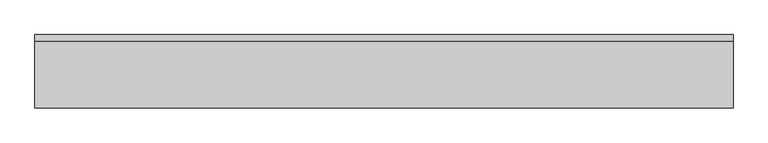
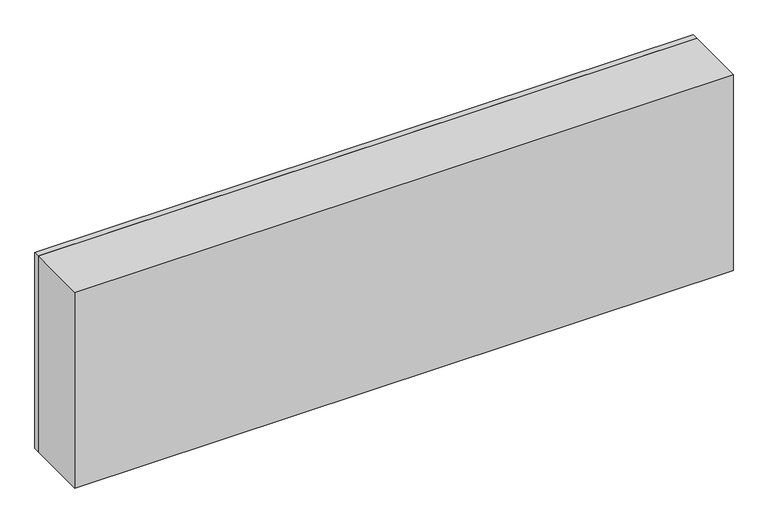
"""IFC4 building model written with IfcOpenShell, lengths in millimetres: furniture geometry, OD_CW_Upper Cabinet : OD_CW_Upper Cabinet."""

from ifc_helpers import new_model, si_unit, frame, origin, place, context, project, spatial, polyline, outline, extrude, source, transform, mapped, element, save


def furniture_1d5eec91(model_context):
    return source(origin(), model_context, "Body", "SweptSolid", [
        extrude(outline(polyline([(18.7377049, -330.2), (18.7377049, -304.8), (2923.5832917, -304.8), (2923.5832917, -330.2), (18.7377049, -330.2)])), frame((0.0, 0.0, 1524.0), z_axis=(0.0, 0.0, 1.0), x_axis=(1.0, 0.0, 0.0)), (0.0, 0.0, 1.0), 914.4),
        extrude(outline(polyline([(18.7377049, -609.6), (18.7377049, -330.2), (2923.5832917, -330.2), (2923.5832917, -609.6), (18.7377049, -609.6)])), frame((0.0, 0.0, 1524.0), z_axis=(0.0, 0.0, 1.0), x_axis=(1.0, 0.0, 0.0)), (0.0, 0.0, 1.0), 914.4),
    ])


if __name__ == "__main__":
    model = new_model("IFC4")
    model_context = context("Model", 3, world=origin())
    ifc_project = project(units=[si_unit("LENGTHUNIT", "METRE", prefix="MILLI")], contexts=[model_context])
    site = spatial("IfcSite", under=ifc_project)
    building = spatial("IfcBuilding", under=site)
    placement = place(None, origin())
    furniture_shape = furniture_1d5eec91(model_context)
    element("IfcFurniture", 1, ObjectType="OD_CW_Upper Cabinet : OD_CW_Upper Cabinet", at=placement, inside=building, context=model_context, shape_type="MappedRepresentation", body=[
        mapped(furniture_shape, transform((0.0, 0.0, 0.0), x_axis=(1.0, 0.0, 0.0), y_axis=(0.0, 1.0, 0.0), z_axis=(0.0, 0.0, 1.0))),
    ])
    save(model, "model.ifc")

# Revit data of these elements
# Type "OD_CW_Upper Cabinet : OD_CW_Upper Cabinet"
#   OD_CW_Width [instance default] = 2' - 2"
#   OD_CW_Off Floor [instance default] = 3' - 2"
#   OD_CW_Length [instance default] = 8' - 0"
#   OD_CW_Height [instance default] = 7' - 0"
#   Depth = 2' - 0"
#   Height = 3' - 0"
#   Width = 4' - 0"
#   OD_CW_Material_Front Panel [instance default] = none
# Element 1 (IfcFurniture, "OD_CW_Upper Cabinet : OD_CW_Upper Cabinet")
#   OD_CW_Width = 1' - 0"
#   OD_CW_Off Floor = 5' - 0"
#   OD_CW_Length = 9' - 6.364"
#   OD_CW_Height = 3' - 0"
#   Materials on its faces: "CASEWORK"
# Materials
#   "CASEWORK": class "Generic", colour RGB 181 181 181, transparency 0, Cost = 0
